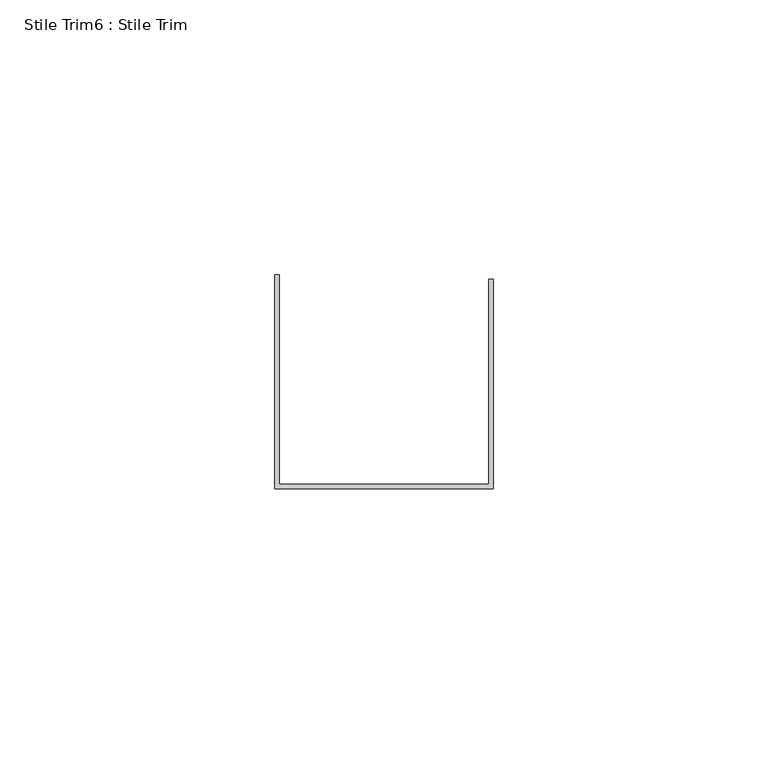
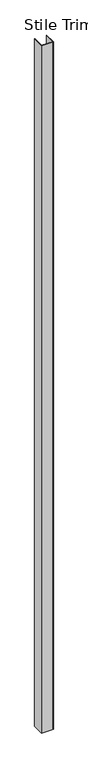
"""IFC4 building model written with IfcOpenShell, lengths in millimetres: proxy geometry, Stile Trim6 : Stile Trim."""

from ifc_helpers import new_model, si_unit, frame, origin, place, context, project, spatial, polyline, outline, extrude, source, transform, mapped, element, save


def stile_trim6_stile_trim_7538b4aa(model_context):
    return source(origin(), model_context, "Body", "SweptSolid", [
        extrude(outline(polyline([(587327.0060739, -531776.5287841), (587327.0060739, -531737.6413841), (587327.7934739, -531737.6413841), (587327.7934739, -531775.7413841), (587365.8934739, -531775.7413841), (587365.8934739, -531738.4287841), (587366.6808739, -531738.4287841), (587366.6808739, -531776.5287841), (587327.0060739, -531776.5287841)])), frame((0.0, 0.0, 11.90625), z_axis=(0.0, 0.0, 1.0), x_axis=(1.0, 0.0, 0.0)), (0.0, 0.0, 1.0), 2426.49375),
    ])


if __name__ == "__main__":
    model = new_model("IFC4")
    model_context = context("Model", 3, world=origin())
    ifc_project = project(units=[si_unit("LENGTHUNIT", "METRE", prefix="MILLI")], contexts=[model_context])
    site = spatial("IfcSite", under=ifc_project)
    building = spatial("IfcBuilding", under=site)
    placement = place(None, origin())
    stile_trim6_stile_trim_shape = stile_trim6_stile_trim_7538b4aa(model_context)
    element("IfcBuildingElementProxy", 1, Name="Stile Trim6 : Stile Trim", ObjectType="Stile Trim6 : Stile Trim", at=placement, inside=building, context=model_context, shape_type="MappedRepresentation", body=[
        mapped(stile_trim6_stile_trim_shape, transform((0.0, 0.0, 0.0), x_axis=(1.0, 0.0, 0.0), y_axis=(0.0, 1.0, 0.0), z_axis=(0.0, 0.0, 1.0))),
    ])
    save(model, "model.ifc")

# Revit data of these elements
# Element 1 (IfcBuildingElementProxy, "Stile Trim6 : Stile Trim")
#   Materials on its faces: "EDGE TRIM BY MTL PANEL MFR."
# Materials
#   "EDGE TRIM BY MTL PANEL MFR.": class "Generic", colour RGB 239 242 240, transparency 0, Cost = 0
